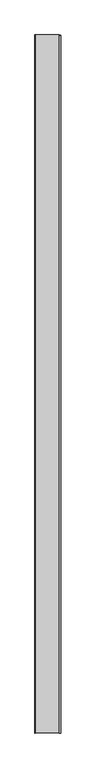
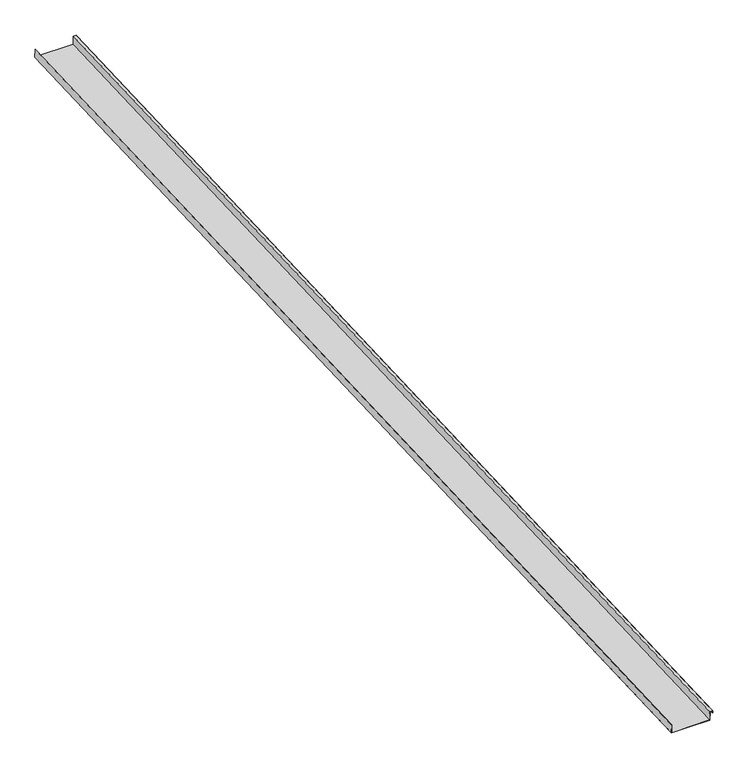
"""IFC4 building model written with IfcOpenShell, lengths in millimetres: proxy geometry, Generic Models 2:Generic Models 2:310765:Generic Models 2:310765 : Generic Models 2:Generic Models 2:310765:201 : Generic Models 2:Generic Models 2:310765:Generic Models 2:310765 : Generic Models 2:Generic Models 2:310765:300385."""

from ifc_helpers import new_model, si_unit, frame, origin, place, context, project, spatial, polyline, outline, extrude, source, transform, mapped, element, save


def generic_models_02c7b9bf(model_context):
    return source(origin(), model_context, "Body", "SweptSolid", [
        extrude(outline(polyline([(50.8, 0.0), (50.8, 14.2875), (41.275, 14.2875), (41.275, 15.875), (52.3875, 15.875), (52.3875, -1.5875), (1.5874999, -1.5875), (1.5874999, -220.6625), (49.2124999, -220.6625), (49.2124999, -222.25), (0.0, -222.25), (0.0, 0.0), (50.8, 0.0)])), frame((579611.7786372, -579052.7217859, 3947.8627097), z_axis=(0.0, 0.9991330730923567, 0.04163054471206783), x_axis=(0.0, -0.04163054471206783, 0.9991330730923567)), (0.0, 0.0, 1.0), 6379.7871853),
    ])


if __name__ == "__main__":
    model = new_model("IFC4")
    model_context = context("Model", 3, world=origin())
    ifc_project = project(units=[si_unit("LENGTHUNIT", "METRE", prefix="MILLI")], contexts=[model_context])
    site = spatial("IfcSite", under=ifc_project)
    building = spatial("IfcBuilding", under=site)
    placement = place(None, origin())
    generic_models_shape = generic_models_02c7b9bf(model_context)
    element("IfcBuildingElementProxy", 1, Name="Generic Models 2:Generic Models 2:310765:Generic Models 2:310765 : Generic Models 2:Generic Models 2:310765:201 : Generic Models 2:Generic Models 2:310765:Generic Models 2:310765 : Generic Models 2:Generic Models 2:310765:300385", ObjectType="Generic Models 2:Generic Models 2:310765:Generic Models 2:310765 : Generic Models 2:Generic Models 2:310765:201 : Generic Models 2:Generic Models 2:310765:Generic Models 2:310765 : Generic Models 2:Generic Models 2:310765:300385", at=placement, inside=building, context=model_context, shape_type="MappedRepresentation", body=[
        mapped(generic_models_shape, transform((0.0, 0.0, 0.0), x_axis=(1.0, 0.0, 0.0), y_axis=(0.0, 1.0, 0.0), z_axis=(0.0, 0.0, 1.0))),
    ])
    save(model, "model.ifc")

# Revit data of these elements
# Type "Generic Models 2:Generic Models 2:310765:Generic Models 2:310765 : Generic Models 2:Generic Models 2:310765:201 : Generic Models 2:Generic Models 2:310765:Generic Models 2:310765 : Generic Models 2:Generic Models 2:310765:300385"
#   NameOverride = "Generic Models 2:Generic Models 2:310765:Generic Models 2:310765 : Generic Models 2:Generic Models 2:310765:300385"
#   ObjectTypeOverride = "Generic Models 2:310765 : Generic Models 2:Generic Models 2:310765"
#   Reference = "Generic Models 2"
#   Tag = "300385"
# Element 1 (IfcBuildingElementProxy, "Generic Models 2:Generic Models 2:310765:Generic Models 2:310765 : Generic Models 2:Generic Models 2:310765:201 : Generic Models 2:Generic Models 2:310765:Generic Models 2:310765 : Generic Models 2:Generic Models 2:310765:300385")
#   Materials on its faces: "THERMAL BROKEN ALUMINUM STOREFRONT FOR POLYCARBONATE"
# Materials
#   "THERMAL BROKEN ALUMINUM STOREFRONT FOR POLYCARBONATE": class "Unassigned", colour RGB 244 244 244, transparency 0, Keynote = "M07611300.01", Cost = 0
